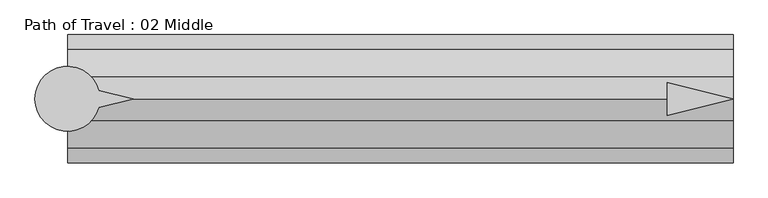
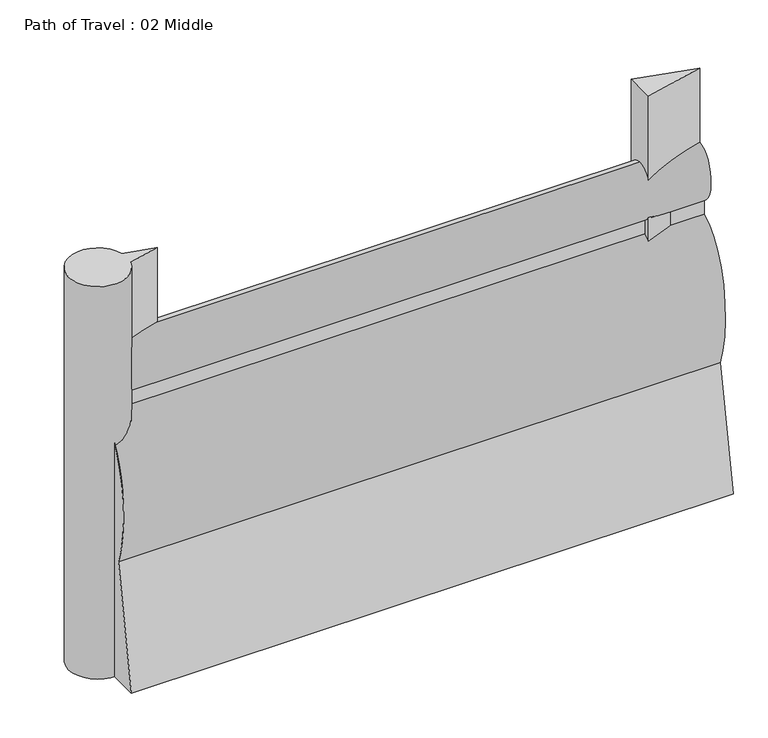
"""IFC4 building model written with IfcOpenShell, lengths in millimetres: proxy geometry, Path of Travel : 02 Middle."""

from ifc_helpers import new_model, si_unit, point, frame, frame_2d, origin, origin_with_axes, place, context, project, spatial, polyline, circle_curve, ellipse_curve, trimmed, segment, composite_curve, outline, extrude, source, transform, mapped, element, save
from ifc_brep_helpers import plane_surface, extruded_surface, advanced_brep


def path_of_travel_02_middle_cb43fae7(model_context):
    return source(origin(), model_context, "Body", "SolidModel", [
        advanced_brep(
        [(227.5554837, 0.0, 1727.2), (227.5554837, 42.9018657, 1436.6534209), (227.5554837, 42.9018657, 1363.4763406), (227.5554837, 184.1186263, 643.4144547), (227.5554837, 297.5699544, 0.0), (227.5554837, 145.6574193, 0.0), (227.5554837, 0.0, 584.2), (227.5554837, -145.6574193, 0.0), (227.5554837, -297.5699544, 0.0), (227.5554837, -184.1186263, 643.4144547), (227.5554837, -42.9018657, 1363.4763406), (227.5554837, -42.9018657, 1436.6534209), (3313.1582246, 0.0, 1727.2), (3313.1582246, -42.9018657, 1436.6534209), (3313.1582246, -42.9018657, 1363.4763406), (3313.1582246, -184.1186263, 643.4144547), (3313.1582246, -297.5699544, 0.0), (3313.1582246, -145.6574193, 0.0), (3313.1582246, 0.0, 584.2), (3313.1582246, 145.6574193, 0.0), (3313.1582246, 297.5699544, 0.0), (3313.1582246, 184.1186263, 643.4144547), (3313.1582246, 42.9018657, 1363.4763406), (3313.1582246, 42.9018657, 1436.6534209)],
        [
            (0, 1, ellipse_curve(frame((227.5554837, 0.0, 1574.8), z_axis=(-1.0, 0.0, 0.0), x_axis=(0.0, 0.0, 1.0)), 152.4, 101.6)),
            (1, 2),
            (2, 3, ellipse_curve(frame((227.5554837, 0.0, 914.4), z_axis=(-1.0, 0.0, 0.0), x_axis=(0.0, 0.0, -1.0)), 457.2, 228.6)),
            (3, 4),
            (4, 5),
            (5, 6),
            (6, 7),
            (7, 8),
            (8, 9),
            (9, 10, ellipse_curve(frame((227.5554837, 0.0, 914.4), z_axis=(-1.0, 0.0, 0.0), x_axis=(0.0, 0.0, -1.0)), 457.2, 228.6)),
            (10, 11),
            (11, 0, ellipse_curve(frame((227.5554837, 0.0, 1574.8), z_axis=(-1.0, 0.0, 0.0), x_axis=(0.0, 0.0, 1.0)), 152.4, 101.6)),
            (12, 13, ellipse_curve(frame((3313.1582246, 0.0, 1574.8), z_axis=(1.0, 0.0, 0.0), x_axis=(0.0, 0.0, 1.0)), 152.4, 101.6)),
            (13, 14),
            (14, 15, ellipse_curve(frame((3313.1582246, 0.0, 914.4), z_axis=(1.0, 0.0, 0.0), x_axis=(0.0, 0.0, -1.0)), 457.2, 228.6)),
            (15, 16),
            (16, 17),
            (17, 18),
            (18, 19),
            (19, 20),
            (20, 21),
            (21, 22, ellipse_curve(frame((3313.1582246, 0.0, 914.4), z_axis=(1.0, 0.0, 0.0), x_axis=(0.0, 0.0, -1.0)), 457.2, 228.6)),
            (22, 23),
            (23, 12, ellipse_curve(frame((3313.1582246, 0.0, 1574.8), z_axis=(1.0, 0.0, 0.0), x_axis=(0.0, 0.0, 1.0)), 152.4, 101.6)),
            (0, 12),
            (23, 1),
            (22, 2),
            (21, 3),
            (20, 4),
            (19, 5),
            (18, 6),
            (17, 7),
            (16, 8),
            (15, 9),
            (14, 10),
            (13, 11),
        ],
        [
            plane_surface(frame((227.5554837, 0.0, 0.0), z_axis=(-1.0, 0.0, 0.0), x_axis=(0.0, 0.0, 1.0))),
            plane_surface(frame((3313.1582246, 0.0, 0.0), z_axis=(1.0, 0.0, 0.0), x_axis=(0.0, 0.0, 1.0))),
            extruded_surface(trimmed(ellipse_curve(frame((3313.1582246, 0.0, 1574.8), z_axis=(-1.0, 0.0, 0.0), x_axis=(0.0, 0.0, 1.0)), 152.4, 101.6), [point((3313.1582246, 0.0, 1727.2))], [point((3313.1582246, 42.9018657, 1436.6534209))], True, "CARTESIAN"), (-3085.6027409, 0.0, 0.0), 3085.6027409),
            plane_surface(frame((227.5554837, 42.9018657, 1436.6534209), z_axis=(0.0, 1.0, 0.0), x_axis=(1.0, 0.0, 0.0))),
            extruded_surface(trimmed(ellipse_curve(frame((3313.1582246, 0.0, 914.4), z_axis=(-1.0, 0.0, 0.0), x_axis=(0.0, 0.0, -1.0)), 457.2, 228.6), [point((3313.1582246, 42.9018657, 1363.4763406))], [point((3313.1582246, 184.1186263, 643.4144547))], True, "CARTESIAN"), (-3085.6027409, 0.0, 0.0), 3085.6027409),
            plane_surface(frame((227.5554837, 184.1186263, 643.4144547), z_axis=(0.0, 0.9848077530122078, 0.1736481776669322), x_axis=(1.0, 0.0, 0.0))),
            plane_surface(frame((227.5554837, 297.5699544, 0.0), z_axis=(0.0, 0.0, -1.0), x_axis=(1.0, 0.0, 0.0))),
            plane_surface(frame((227.5554837, 145.6574193, 0.0), z_axis=(0.0, -0.9702957262760199, -0.2419218955995739), x_axis=(1.0, 0.0, 0.0))),
            plane_surface(frame((227.5554837, 0.0, 584.2), z_axis=(0.0, 0.9702957262759961, -0.24192189559966923), x_axis=(1.0, 0.0, 0.0))),
            plane_surface(frame((227.5554837, -145.6574193, 0.0), z_axis=(0.0, 0.0, -1.0), x_axis=(1.0, 0.0, 0.0))),
            plane_surface(frame((227.5554837, -297.5699544, 0.0), z_axis=(0.0, -0.984807753012208, 0.17364817766693066), x_axis=(1.0, 0.0, 0.0))),
            extruded_surface(trimmed(ellipse_curve(frame((3313.1582246, 0.0, 914.4), z_axis=(-1.0, 0.0, 0.0), x_axis=(0.0, 0.0, -1.0)), 457.2, 228.6), [point((3313.1582246, -184.1186263, 643.4144547))], [point((3313.1582246, -42.9018657, 1363.4763406))], True, "CARTESIAN"), (-3085.6027409, 0.0, 0.0), 3085.6027409),
            plane_surface(frame((227.5554837, -42.9018657, 1363.4763406), z_axis=(0.0, -1.0, 0.0), x_axis=(1.0, 0.0, 0.0))),
            extruded_surface(trimmed(ellipse_curve(frame((3313.1582246, 0.0, 1574.8), z_axis=(-1.0, 0.0, 0.0), x_axis=(0.0, 0.0, 1.0)), 152.4, 101.6), [point((3313.1582246, -42.9018657, 1436.6534209))], [point((3313.1582246, 0.0, 1727.2))], True, "CARTESIAN"), (-3085.6027409, 0.0, 0.0), 3085.6027409),
        ],
        [
            (0, [[1, 2, 3, 4, 5, 6, 7, 8, 9, 10, 11, 12]]),
            (1, [[13, 14, 15, 16, 17, 18, 19, 20, 21, 22, 23, 24]]),
            (2, [[-1, 25, -24, 26]]),
            (3, [[-2, -26, -23, 27]]),
            (4, [[-3, -27, -22, 28]]),
            (5, [[-4, -28, -21, 29]]),
            (6, [[-5, -29, -20, 30]]),
            (7, [[-6, -30, -19, 31]]),
            (8, [[-7, -31, -18, 32]]),
            (9, [[-8, -32, -17, 33]]),
            (10, [[-9, -33, -16, 34]]),
            (11, [[-10, -34, -15, 35]]),
            (12, [[-11, -35, -14, 36]]),
            (13, [[-12, -36, -13, -25]]),
        ],
    ),
        extrude(outline(polyline([(3007.153078, 76.2006338), (3313.1582246, 0.0), (3007.153078, -76.2006338), (3007.153078, 76.2006338)])), origin_with_axes(), (0.0, 0.0, 1.0), 2129.5973753),
        extrude(outline(composite_curve([segment(polyline([(372.7837828, 39.4440225), (531.182385, 0.0), (372.7837828, -39.4440225)]), True, "CONTINUOUS"), segment(trimmed(circle_curve(frame_2d((227.2200886, 0.0)), 150.8131956), [point((372.7837828, -39.4440225))], [point((372.7837828, 39.4440225))], False, "CARTESIAN"), True, "CONTINUOUS")], self_intersect=False)), origin_with_axes(), (0.0, 0.0, 1.0), 2129.5973753),
    ])


if __name__ == "__main__":
    model = new_model("IFC4")
    model_context = context("Model", 3, world=origin())
    ifc_project = project(units=[si_unit("LENGTHUNIT", "METRE", prefix="MILLI")], contexts=[model_context])
    site = spatial("IfcSite", under=ifc_project)
    building = spatial("IfcBuilding", under=site)
    placement = place(None, origin())
    path_of_travel_02_middle_shape = path_of_travel_02_middle_cb43fae7(model_context)
    element("IfcBuildingElementProxy", 1, Name="Path of Travel : 02 Middle", ObjectType="Path of Travel : 02 Middle", at=placement, inside=building, context=model_context, shape_type="MappedRepresentation", body=[
        mapped(path_of_travel_02_middle_shape, transform((0.0, 0.0, 0.0), x_axis=(1.0, 0.0, 0.0), y_axis=(0.0, 1.0, 0.0), z_axis=(0.0, 0.0, 1.0))),
    ])
    save(model, "model.ifc")

# Revit data of these elements
# Type "Path of Travel : 02 Middle"
#   Path of Egress [instance default] = 4' - 0"
#   built-in parameter 1001306 [instance default] = 4 (stored number, unit not read)
#   Dot at Start = no
#   Arrow in Middle = yes
#   Arrow at End = no
#   Egress Path = none
# Element 1 (IfcBuildingElementProxy, "Path of Travel : 02 Middle")
#   Path of Egress = 10' - 1.48042"
#   built-in parameter 1001306 = 10.1234 (stored number, unit not read)
